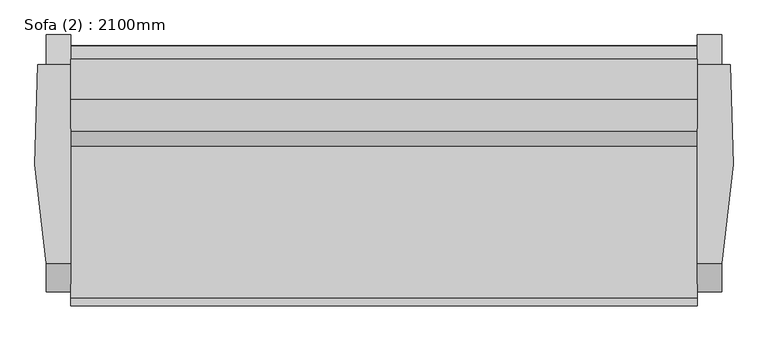
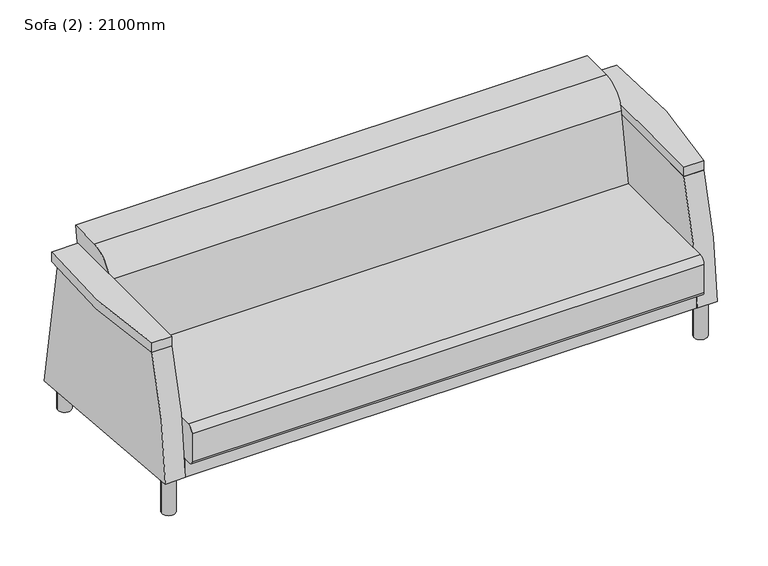
"""IFC4 building model written with IfcOpenShell, lengths in millimetres: furniture geometry, Sofa (2) : 2100mm."""

from ifc_helpers import new_model, si_unit, point, frame, frame_2d, origin, origin_with_axes, place, context, project, spatial, polyline, circle_curve, trimmed, segment, composite_curve, outline, extrude, source, transform, mapped, element, save


def sofa_2_2100mm_9ba79c6e(model_context):
    return source(origin(), model_context, "Body", "SweptSolid", [
        extrude(outline(composite_curve([segment(trimmed(circle_curve(frame_2d((-733.29375, -53.0901639)), 25.4), [point((-758.69375, -53.0901639))], [point((-707.89375, -53.0901639))], False, "CARTESIAN"), True, "CONTINUOUS"), segment(trimmed(circle_curve(frame_2d((-733.29375, -53.0901639)), 25.4), [point((-707.89375, -53.0901639))], [point((-758.69375, -53.0901639))], False, "CARTESIAN"), True, "CONTINUOUS")], self_intersect=False)), origin_with_axes(), (0.0, 0.0, 1.0), 148.43125),
        extrude(outline(composite_curve([segment(trimmed(circle_curve(frame_2d((-733.29375, 632.7098361)), 25.4), [point((-758.69375, 632.7098361))], [point((-707.89375, 632.7098361))], False, "CARTESIAN"), True, "CONTINUOUS"), segment(trimmed(circle_curve(frame_2d((-733.29375, 632.7098361)), 25.4), [point((-707.89375, 632.7098361))], [point((-758.69375, 632.7098361))], False, "CARTESIAN"), True, "CONTINUOUS")], self_intersect=False)), origin_with_axes(), (0.0, 0.0, 1.0), 148.43125),
        extrude(outline(composite_curve([segment(trimmed(circle_curve(frame_2d((1290.50625, 632.7098361)), 25.4), [point((1265.10625, 632.7098361))], [point((1315.90625, 632.7098361))], False, "CARTESIAN"), True, "CONTINUOUS"), segment(trimmed(circle_curve(frame_2d((1290.50625, 632.7098361)), 25.4), [point((1315.90625, 632.7098361))], [point((1265.10625, 632.7098361))], False, "CARTESIAN"), True, "CONTINUOUS")], self_intersect=False)), origin_with_axes(), (0.0, 0.0, 1.0), 148.43125),
        extrude(outline(composite_curve([segment(trimmed(circle_curve(frame_2d((1290.50625, -53.0901639)), 25.4), [point((1265.10625, -53.0901639))], [point((1315.90625, -53.0901639))], False, "CARTESIAN"), True, "CONTINUOUS"), segment(trimmed(circle_curve(frame_2d((1290.50625, -53.0901639)), 25.4), [point((1315.90625, -53.0901639))], [point((1265.10625, -53.0901639))], False, "CARTESIAN"), True, "CONTINUOUS")], self_intersect=False)), origin_with_axes(), (0.0, 0.0, 1.0), 148.43125),
        extrude(outline(polyline([(1252.40625, 668.3047863), (1252.40625, -93.6952137), (-695.19375, -93.6952137), (-695.19375, 668.3047863), (1252.40625, 668.3047863)])), frame((0.0, 0.0, 148.0509954), z_axis=(0.0, 0.0, 1.0), x_axis=(1.0, 0.0, 0.0)), (0.0, 0.0, 1.0), 76.2),
        extrude(outline(composite_curve([segment(polyline([(-9.3943348, 626.0203985), (608.6917937, 626.0203985), (701.7619204, 79.3588346), (-97.7900405, 149.3105671)]), True, "CONTINUOUS"), segment(trimmed(circle_curve(frame_2d((1499.9783711, 99.5888442)), 1598.5418814), [point((-97.7900405, 149.3105671))], [point((-9.3943348, 626.0203985))], False, "CARTESIAN"), True, "CONTINUOUS")], self_intersect=False)), frame((-771.39375, 0.0, 0.0), z_axis=(1.0, 0.0, 0.0), x_axis=(0.0, 1.0, 0.0)), (0.0, 0.0, 1.0), 76.2),
        extrude(outline(composite_curve([segment(polyline([(701.7619204, 79.3588346), (-97.7900405, 149.3105671)]), True, "CONTINUOUS"), segment(trimmed(circle_curve(frame_2d((1499.9783711, 99.5888442)), 1598.5418814), [point((-97.7900405, 149.3105671))], [point((-9.3943348, 626.0203985))], False, "CARTESIAN"), True, "CONTINUOUS"), segment(polyline([(-9.3943348, 626.0203985), (608.6917937, 626.0203985), (701.7619204, 79.3588346)]), True, "CONTINUOUS")], self_intersect=False)), frame((1252.40625, 0.0, 0.0), z_axis=(1.0, 0.0, 0.0), x_axis=(0.0, 1.0, 0.0)), (0.0, 0.0, 1.0), 76.2),
        extrude(outline(composite_curve([segment(trimmed(circle_curve(frame_2d((-116.5901639, 351.2509954)), 25.4), [point((-141.9901639, 351.2509954))], [point((-116.5901639, 376.6509954))], False, "CARTESIAN"), True, "CONTINUOUS"), segment(polyline([(-116.5901639, 376.6509954), (355.3895541, 376.6509954), (402.1988177, 642.1195211)]), True, "CONTINUOUS"), segment(trimmed(circle_curve(frame_2d((502.2552854, 624.4768662)), 101.6), [point((402.1988177, 642.1195211))], [point((502.2552854, 726.0768662))], False, "CARTESIAN"), True, "CONTINUOUS"), segment(polyline([(502.2552854, 726.0768662), (626.3344485, 726.0768662), (609.5377828, 620.1719187), (667.6541767, 224.2509954), (-126.1151639, 224.2509954)]), True, "CONTINUOUS"), segment(trimmed(circle_curve(frame_2d((-126.1151639, 240.1259954)), 15.875), [point((-126.1151639, 224.2509954))], [point((-141.9901639, 240.1259954))], False, "CARTESIAN"), True, "CONTINUOUS"), segment(polyline([(-141.9901639, 240.1259954), (-141.9901639, 351.2509954)]), True, "CONTINUOUS")], self_intersect=False)), frame((-695.19375, 0.0, 0.0), z_axis=(1.0, 0.0, 0.0), x_axis=(0.0, 1.0, 0.0)), (0.0, 0.0, 1.0), 1947.6),
        extrude(outline(composite_curve([segment(polyline([(-695.19375, -9.3943348), (-771.39375, -9.3943348)]), True, "CONTINUOUS"), segment(trimmed(circle_curve(frame_2d((1362.7527561, 387.8725201)), 2170.8068232), [point((-771.39375, -9.3943348))], [point((-796.79375, 608.6917935))], False, "CARTESIAN"), True, "CONTINUOUS"), segment(polyline([(-796.79375, 608.6917935), (-695.19375, 608.6917935), (-695.19375, -9.3943348)]), True, "CONTINUOUS")], self_intersect=False)), frame((0.0, 0.0, 626.0203985), z_axis=(0.0, 0.0, 1.0), x_axis=(1.0, 0.0, 0.0)), (0.0, 0.0, 1.0), 38.1),
        extrude(outline(composite_curve([segment(polyline([(1252.40625, -9.3943348), (1252.40625, 608.9395268), (1353.9809043, 608.9395268)]), True, "CONTINUOUS"), segment(trimmed(circle_curve(frame_2d((-805.5402561, 387.8725201)), 2170.8068232), [point((1353.9809043, 608.9395268))], [point((1328.60625, -9.3943348))], False, "CARTESIAN"), True, "CONTINUOUS"), segment(polyline([(1328.60625, -9.3943348), (1252.40625, -9.3943348)]), True, "CONTINUOUS")], self_intersect=False)), frame((0.0, 0.0, 626.0203985), z_axis=(0.0, 0.0, 1.0), x_axis=(1.0, 0.0, 0.0)), (0.0, 0.0, 1.0), 38.1),
    ])


if __name__ == "__main__":
    model = new_model("IFC4")
    model_context = context("Model", 3, world=origin())
    ifc_project = project(units=[si_unit("LENGTHUNIT", "METRE", prefix="MILLI")], contexts=[model_context])
    site = spatial("IfcSite", under=ifc_project)
    building = spatial("IfcBuilding", under=site)
    placement = place(None, origin())
    sofa_2_2100mm_shape = sofa_2_2100mm_9ba79c6e(model_context)
    element("IfcFurniture", 1, ObjectType="Sofa (2) : 2100mm", at=placement, inside=building, context=model_context, shape_type="MappedRepresentation", body=[
        mapped(sofa_2_2100mm_shape, transform((0.0, 0.0, 0.0), x_axis=(1.0, 0.0, 0.0), y_axis=(0.0, 1.0, 0.0), z_axis=(0.0, 0.0, 1.0))),
    ])
    save(model, "model.ifc")

# Revit data of these elements
# Type "Sofa (2) : 2100mm"
#   Keynote = "N"
#   Length = 2.1 m
#   Material Sofa = Textile - Linen, Smooth
#   Material Frame = Metal - Chrome
#   Assembly Code = ""
# Element 1 (IfcFurniture, "Sofa (2) : 2100mm")
#   Materials on its faces: "Textile - Linen, Smooth", "Metal - Chrome"
# Materials
#   "Textile - Linen, Smooth": class "Fabric", colour RGB 249 239 230, transparency 0
#   "Metal - Chrome": class "Metal", colour RGB 247 247 247, transparency 0
